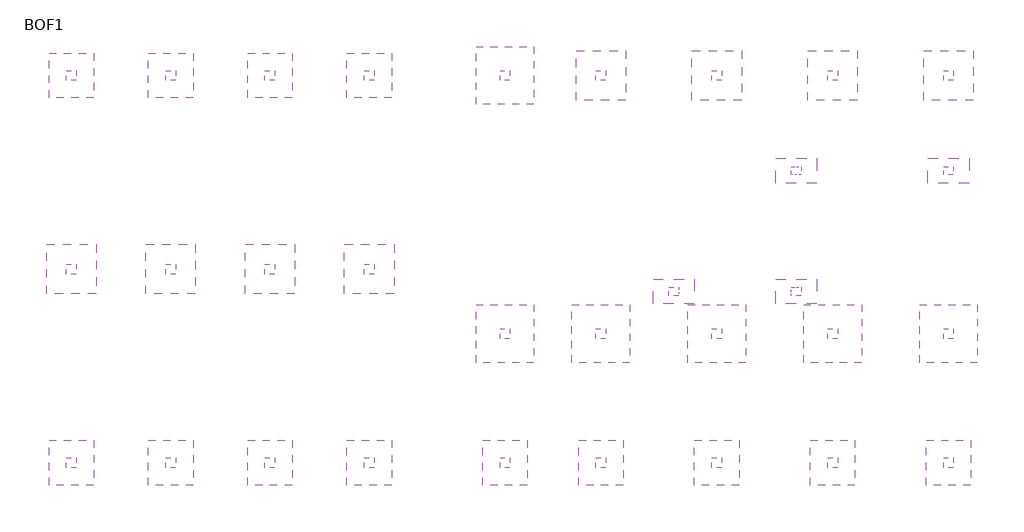
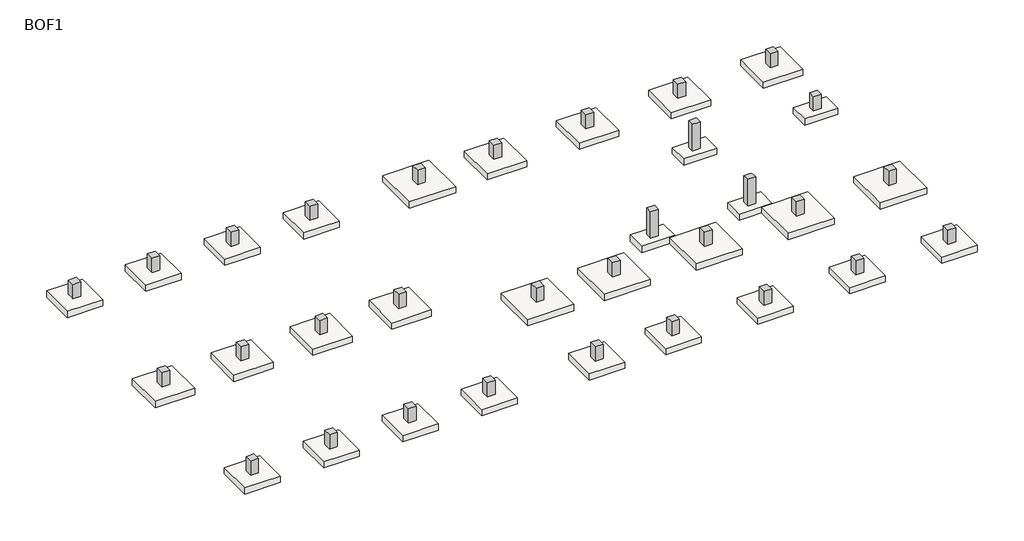
# One storey: 31 columns, 31 slabs.
"""IFC4 building model written with IfcOpenShell, lengths in millimetres."""

import ifcopenshell
import ifcopenshell.guid

model = None  # the IFC model being written
_history = None  # IfcOwnerHistory: only IFC2X3 demands one
_inside = {}  # id of a spatial element -> (the spatial element, [elements in it])
_under = {}  # id of a project, library or spatial element -> (it, [spatial elements below it])
_declared = {}  # id of a project -> (the project, [libraries it declares])
_typed = {}  # id of a type object -> (the type object, [elements of that type])
_made_of = {}  # id of a material, layer set ... -> (it, [elements and type objects made of it])


def new_model(schema):
    """Start an empty IFC model of exactly this schema.

    Asked for "IFC4X3", IfcOpenShell would pick the latest addendum, in which some entities
    have other attributes; the version numbers below select the first issue.
    IFC2X3 requires an IfcOwnerHistory on every rooted entity: one is made here for all.
    """
    global model, _history
    if schema == "IFC4X3":
        model = ifcopenshell.file(schema_version=(4, 3, 0, 0))
    else:
        model = ifcopenshell.file(schema=schema)
    _inside.clear()
    _under.clear()
    _declared.clear()
    _typed.clear()
    _made_of.clear()
    _history = None
    if model.schema == "IFC2X3":
        org = make("IfcOrganization", Name="unknown")
        user = make(
            "IfcPersonAndOrganization",
            ThePerson=make("IfcPerson", FamilyName="unknown"),
            TheOrganization=org,
        )
        app = make(
            "IfcApplication",
            ApplicationDeveloper=org,
            Version="unknown",
            ApplicationFullName="unknown",
            ApplicationIdentifier="unknown",
        )
        _history = make(
            "IfcOwnerHistory",
            OwningUser=user,
            OwningApplication=app,
            ChangeAction="ADDED",
            CreationDate=0,
        )
    return model


def make(cls, **values):
    """One entity of the class cls with the attributes given. An attribute that is None is left unset."""
    return model.create_entity(
        cls, **{name: value for name, value in values.items() if value is not None}
    )


def rooted(cls, **values):
    """An entity with a GlobalId (a new one), such as an element, a storey or a relation."""
    return make(cls, GlobalId=ifcopenshell.guid.new(), OwnerHistory=_history, **values)


def si_unit(unit_type, name, prefix=None):
    """IfcSIUnit, for example si_unit("LENGTHUNIT", "METRE", prefix="MILLI")."""
    return make("IfcSIUnit", UnitType=unit_type, Prefix=prefix, Name=name)


def assignment(units):
    """IfcUnitAssignment: the units of a project."""
    return None if units is None else make("IfcUnitAssignment", Units=units)


def point(xyz):
    """IfcCartesianPoint."""
    return None if xyz is None else make("IfcCartesianPoint", Coordinates=xyz)


def direction(xyz):
    """IfcDirection."""
    return None if xyz is None else make("IfcDirection", DirectionRatios=xyz)


def frame(location, z_axis=None, x_axis=None):
    """IfcAxis2Placement3D, a coordinate frame: its origin and axes. An axis left out is left unset."""
    return make(
        "IfcAxis2Placement3D",
        Location=point(location),
        Axis=direction(z_axis),
        RefDirection=direction(x_axis),
    )


def origin():
    """The frame at (0, 0, 0) with its axes left unset."""
    return frame((0.0, 0.0, 0.0))


def place(relative_to, where):
    """IfcLocalPlacement: puts the frame where relative to a parent placement (None: the world)."""
    return make(
        "IfcLocalPlacement", PlacementRelTo=relative_to, RelativePlacement=where
    )


def context(
    kind, dimensions, precision=None, world=None, true_north=None, identifier=None
):
    """IfcGeometricRepresentationContext, for example the 3D "Model" context."""
    return make(
        "IfcGeometricRepresentationContext",
        ContextIdentifier=identifier,
        ContextType=kind,
        CoordinateSpaceDimension=dimensions,
        Precision=precision,
        WorldCoordinateSystem=world,
        TrueNorth=true_north,
    )


def project(units=None, contexts=None):
    """IfcProject with its units and contexts."""
    return rooted(
        "IfcProject",
        Name="project",
        RepresentationContexts=contexts,
        UnitsInContext=assignment(units),
    )


def spatial(cls, under=None, at=None, **own):
    """A site, building, storey or space (cls), placed at a placement, below another one or the project."""
    s = rooted(cls, ObjectPlacement=at, **own)
    if under is not None:
        _under.setdefault(under.id(), (under, []))[1].append(s)
    return s


def polyline(points):
    """IfcPolyline through the points."""
    return make("IfcPolyline", Points=[point(p) for p in points])


def outline(outer, holes=None, kind="AREA"):
    """IfcArbitraryClosedProfileDef: a profile drawn as a closed curve; with holes, ...WithVoids."""
    if holes is None:
        return make("IfcArbitraryClosedProfileDef", ProfileType=kind, OuterCurve=outer)
    return make(
        "IfcArbitraryProfileDefWithVoids",
        ProfileType=kind,
        OuterCurve=outer,
        InnerCurves=holes,
    )


def extrude(swept, where, along, depth):
    """IfcExtrudedAreaSolid: the profile swept, set in the frame where, extruded along a direction by depth."""
    return make(
        "IfcExtrudedAreaSolid",
        SweptArea=swept,
        Position=where,
        ExtrudedDirection=direction(along),
        Depth=depth,
    )


def faces_of(points, faces, orient=None, outer=None):
    """IfcFace entities. A face is a list of loops; a loop is a list of indices into points, from 0.

    orient and outer hold one flag for each loop. By default every Orientation is true, the
    first loop of a face is its IfcFaceOuterBound and the others are IfcFaceBound.
    """
    made = []
    for i, loops in enumerate(faces):
        bounds = []
        for j, loop in enumerate(loops):
            is_outer = j == 0 if outer is None else outer[i][j]
            bounds.append(
                make(
                    "IfcFaceOuterBound" if is_outer else "IfcFaceBound",
                    Bound=make("IfcPolyLoop", Polygon=[points[k] for k in loop]),
                    Orientation=True if orient is None else orient[i][j],
                )
            )
        made.append(make("IfcFace", Bounds=bounds))
    return made


def faceted_brep(points, faces, orient=None, outer=None, voids=None):
    """IfcFacetedBrep: a solid bounded by flat faces; with voids (closed shells), ...WithVoids."""
    shared = [point(p) for p in points]
    hull = make("IfcClosedShell", CfsFaces=faces_of(shared, faces, orient, outer))
    if voids is None:
        return make("IfcFacetedBrep", Outer=hull)
    return make(
        "IfcFacetedBrepWithVoids",
        Outer=hull,
        Voids=[
            make(cls, CfsFaces=faces_of(shared, fs, o, b)) for cls, fs, o, b in voids
        ],
    )


def shape(context_of_items, identifier, shape_type, items):
    """IfcShapeRepresentation: the items that make up one representation, for example the "Body"."""
    return make(
        "IfcShapeRepresentation",
        ContextOfItems=context_of_items,
        RepresentationIdentifier=identifier,
        RepresentationType=shape_type,
        Items=items,
    )


def source(mapping_origin, context_of_items, identifier, shape_type, items):
    """IfcRepresentationMap: a shape defined once, which mapped items show again and again."""
    return make(
        "IfcRepresentationMap",
        MappingOrigin=mapping_origin,
        MappedRepresentation=shape(context_of_items, identifier, shape_type, items),
    )


def transform(
    local_origin,
    x_axis=None,
    y_axis=None,
    z_axis=None,
    scale=None,
    scale2=None,
    scale3=None,
    uniform=True,
):
    """IfcCartesianTransformationOperator3D, or its non-uniform kind. x_axis, y_axis, z_axis: its Axis1, 2, 3."""
    if uniform:
        return make(
            "IfcCartesianTransformationOperator3D",
            Axis1=direction(x_axis),
            Axis2=direction(y_axis),
            LocalOrigin=point(local_origin),
            Scale=scale,
            Axis3=direction(z_axis),
        )
    return make(
        "IfcCartesianTransformationOperator3DnonUniform",
        Axis1=direction(x_axis),
        Axis2=direction(y_axis),
        LocalOrigin=point(local_origin),
        Scale=scale,
        Axis3=direction(z_axis),
        Scale2=scale2,
        Scale3=scale3,
    )


def mapped(mapping_source, mapping_target):
    """IfcMappedItem: shows the shape of a source again, moved by a transform."""
    return make(
        "IfcMappedItem", MappingSource=mapping_source, MappingTarget=mapping_target
    )


def made_of(thing, what):
    """Note that an element or type object is made of a material, layer set ...; save() writes the relation."""
    if what is not None:
        _made_of.setdefault(what.id(), (what, []))[1].append(thing)
    return thing


def element(
    cls,
    number,
    at=None,
    inside=None,
    cuts=None,
    type_object=None,
    material=None,
    context=None,
    identifier="Body",
    shape_type=None,
    held_by="IfcProductDefinitionShape",
    body=None,
    shapes=None,
    **own,
):
    """One element of the class cls, such as IfcWall. Its Tag is "e" and its number.

    at: its placement. inside: the storey or other place that contains it. cuts: it is an
    opening in that element (IfcRelVoidsElement). A single representation is given by context,
    identifier, shape_type and body (its items); several are given by shapes. held_by: the class
    of the entity that holds the representations. save() writes the other relations.
    """
    e = rooted(cls, Tag="e%d" % number, ObjectPlacement=at, **own)
    if body is not None:
        shapes = [shape(context, identifier, shape_type, body)]
    if shapes is not None:
        e.Representation = make(held_by, Representations=shapes)
    if inside is not None:
        _inside.setdefault(inside.id(), (inside, []))[1].append(e)
    if cuts is not None:
        rooted(
            "IfcRelVoidsElement", RelatingBuildingElement=cuts, RelatedOpeningElement=e
        )
    if type_object is not None:
        _typed.setdefault(type_object.id(), (type_object, []))[1].append(e)
    return made_of(e, material)


def aggregate(whole, parts):
    """IfcRelAggregates: a whole, such as a stair, and the parts it consists of."""
    return rooted("IfcRelAggregates", RelatingObject=whole, RelatedObjects=parts)


def save(model, path):
    """Write the relations noted so far, then the file.

    IfcRelAggregates (storeys below a building ...), IfcRelContainedInSpatialStructure (elements
    in a storey), IfcRelDefinesByType, IfcRelAssociatesMaterial and IfcRelDeclares: one each for
    every whole, place, type object, material and project.
    """
    for whole, parts in _under.values():
        aggregate(whole, parts)
    for where, things in _inside.values():
        rooted(
            "IfcRelContainedInSpatialStructure",
            RelatedElements=things,
            RelatingStructure=where,
        )
    for kind, things in _typed.values():
        rooted("IfcRelDefinesByType", RelatedObjects=things, RelatingType=kind)
    for what, things in _made_of.values():
        rooted("IfcRelAssociatesMaterial", RelatedObjects=things, RelatingMaterial=what)
    for by, libraries in _declared.values():
        rooted("IfcRelDeclares", RelatingContext=by, RelatedDefinitions=libraries)
    model.write(path)


def foundation_rectangular_non_pile_db20e422(model_context):
    return source(origin(), model_context, "Body", "SweptSolid", [
        extrude(outline(polyline([(1350.0, 1350.0), (1350.0, -1350.0), (-1350.0, -1350.0), (-1350.0, 1350.0), (1350.0, 1350.0)])), frame((0.0, 0.0, -500.0), z_axis=(0.0, 0.0, 1.0), x_axis=(1.0, 0.0, 0.0)), (0.0, 0.0, 1.0), 500.0),
    ])


def foundation_rectangular_non_pile_a43cc813(model_context):
    return source(origin(), model_context, "Body", "SweptSolid", [
        extrude(outline(polyline([(1500.0, 1500.0), (1500.0, -1500.0), (-1500.0, -1500.0), (-1500.0, 1500.0), (1500.0, 1500.0)])), frame((0.0, 0.0, -500.0), z_axis=(0.0, 0.0, 1.0), x_axis=(1.0, 0.0, 0.0)), (0.0, 0.0, 1.0), 500.0),
    ])


def foundation_rectangular_non_pile_20b31725(model_context):
    return source(origin(), model_context, "Body", "SweptSolid", [
        extrude(outline(polyline([(1750.0, 1750.0), (1750.0, -1750.0), (-1750.0, -1750.0), (-1750.0, 1750.0), (1750.0, 1750.0)])), frame((0.0, 0.0, -500.0), z_axis=(0.0, 0.0, 1.0), x_axis=(1.0, 0.0, 0.0)), (0.0, 0.0, 1.0), 500.0),
    ])


def foundation_rectangular_non_pile_907a7f09(model_context):
    return source(origin(), model_context, "Body", "SweptSolid", [
        extrude(outline(polyline([(1250.0, 750.0), (1250.0, -750.0), (-1250.0, -750.0), (-1250.0, 750.0), (1250.0, 750.0)])), frame((0.0, 0.0, -500.0), z_axis=(0.0, 0.0, 1.0), x_axis=(1.0, 0.0, 0.0)), (0.0, 0.0, 1.0), 500.0),
    ])


model = new_model("IFC4")

# Units and contexts
model_context = context("Model", 3, world=origin())
ifc_project = project(units=[si_unit("LENGTHUNIT", "METRE", prefix="MILLI")], contexts=[model_context])

# Site, building, storey
site = spatial("IfcSite", under=ifc_project)
building = spatial("IfcBuilding", under=site)
storey = spatial("IfcBuildingStorey", under=building, Name="BOF1", Elevation=88650.0)

# Columns
placement = place(None, origin())
element("IfcColumn", 1, ObjectType="RC_Column_Rectangular : H_SC_AR_S15_UG PED_Bit_600x500_PD1", at=placement, inside=storey, context=model_context, shape_type="Brep", body=[
    faceted_brep([(36700.0, -9400.0, 95900.0), (36100.0, -9400.0, 95900.0), (36100.0, -8900.0, 95900.0), (36700.0, -8900.0, 95900.0), (36700.0, -9400.0, 98049.9618634), (36100.0, -9400.0, 98049.9618634), (36700.0, -9400.0, 97049.9618634), (36100.0, -8900.0, 98049.9618634), (36700.0, -8900.0, 98049.9618634), (36700.0, -9200.0, 98049.9618634)], [[[0, 1, 2, 3]], [[4, 5, 1, 0, 6]], [[5, 7, 2, 1]], [[7, 8, 3, 2]], [[8, 9, 4, 6, 0, 3]], [[4, 9, 8, 7, 5]]]),
])
element("IfcColumn", 2, ObjectType="RC_Column_Rectangular : H_SC_AR_S15_UG PED_Bit_600x500_PD1", at=placement, inside=storey, context=model_context, shape_type="Brep", body=[
    faceted_brep([(44100.0, -9400.0, 95900.0), (43500.0, -9400.0, 95900.0), (43500.0, -8900.0, 95900.0), (44100.0, -8900.0, 95900.0), (44100.0, -9400.0, 98049.9618634), (43500.0, -9400.0, 98049.9618634), (43500.0, -9400.0, 97049.9618634), (43500.0, -9200.0, 98049.9618634), (43500.0, -8900.0, 98049.9618634), (43600.0, -8900.0, 98049.9618634), (43800.0, -8900.0, 98049.9618634), (44100.0, -8900.0, 98049.9618634)], [[[0, 1, 2, 3]], [[4, 5, 6, 1, 0]], [[5, 7, 8, 2, 1, 6]], [[8, 9, 10, 11, 3, 2]], [[11, 4, 0, 3]], [[4, 11, 10, 9, 8, 7, 5]]]),
])
element("IfcColumn", 3, ObjectType="RC_Column_Rectangular : H_SC_AR_S15_UG PED_Bit_600x500_PD1", at=placement, inside=storey, context=model_context, shape_type="Brep", body=[
    faceted_brep([(44100.0, -2100.0, 95900.0), (43500.0, -2100.0, 95900.0), (43500.0, -1600.0, 95900.0), (44100.0, -1600.0, 95900.0), (44100.0, -2100.0, 98049.9618634), (43800.0, -2100.0, 98049.9618634), (43600.0, -2100.0, 98049.9618634), (43500.0, -2100.0, 98049.9618634), (43500.0, -2100.0, 97049.9618634), (43500.0, -2100.0, 96399.9618634), (44100.0, -2100.0, 96399.9618634), (44100.0, -2100.0, 97049.9618634), (43500.0, -1600.0, 98049.9618634), (43500.0, -1600.0, 97049.9618634), (43500.0, -1600.0, 96399.9618634), (43600.0, -1600.0, 98049.9618634), (43800.0, -1600.0, 98049.9618634), (44100.0, -1600.0, 98049.9618634), (44100.0, -1600.0, 97049.9618634), (44100.0, -1600.0, 96399.9618634)], [[[0, 1, 2, 3]], [[4, 5, 6, 7, 8, 9, 1, 0, 10, 11]], [[7, 12, 13, 14, 2, 1, 9, 8]], [[12, 15, 16, 17, 18, 19, 3, 2, 14, 13]], [[17, 4, 11, 10, 0, 3, 19, 18]], [[4, 17, 16, 15, 12, 7, 6, 5]]]),
])
element("IfcColumn", 4, ObjectType="RC_Column_Rectangular : H_SC_AR_S15_UG PED_Bit_600x500_PD1A", at=placement, inside=storey, context=model_context, shape_type="Brep", body=[
    faceted_brep([(53300.0, -2100.0, 95900.0), (52700.0, -2100.0, 95900.0), (52700.0, -1600.0, 95900.0), (53300.0, -1600.0, 95900.0), (53300.0, -2100.0, 97049.9618634), (52700.0, -2100.0, 97049.9618634), (52700.0, -2100.0, 96399.9618634), (53300.0, -2100.0, 96399.9618634), (52700.0, -1600.0, 97049.9618634), (52700.0, -1600.0, 96399.9618634), (53300.0, -1600.0, 97049.9618634), (53300.0, -1600.0, 96399.9618634)], [[[0, 1, 2, 3]], [[4, 5, 6, 1, 0, 7]], [[5, 8, 9, 2, 1, 6]], [[8, 10, 11, 3, 2, 9]], [[10, 4, 7, 0, 3, 11]], [[4, 10, 8, 5]]]),
])
element("IfcColumn", 5, ObjectType="RC_Column_Rectangular : H_SC_AR S15_UG Ped_C1 600x600", at=placement, inside=storey, context=model_context, shape_type="SweptSolid", body=[
    extrude(outline(polyline([(300.0, -19200.0), (300.0, -19800.0), (-300.0, -19800.0), (-300.0, -19200.0), (300.0, -19200.0)])), frame((0.0, 0.0, 95900.0), z_axis=(0.0, 0.0, 1.0), x_axis=(1.0, 0.0, 0.0)), (0.0, 0.0, 1.0), 1149.9618634),
])
element("IfcColumn", 6, ObjectType="RC_Column_Rectangular : H_SC_AR S15_UG Ped_C1 600x600", at=placement, inside=storey, context=model_context, shape_type="Brep", body=[
    faceted_brep([(26500.0, -11400.0, 95900.0), (26500.0, -12000.0, 95900.0), (25900.0, -12000.0, 95900.0), (25900.0, -11400.0, 95900.0), (26500.0, -11400.0, 97049.9618634), (26500.0, -12000.0, 97049.9618634), (25900.0, -12000.0, 97049.9618634), (25900.0, -11400.0, 97049.9618634), (25900.0, -11400.0, 96849.9618634)], [[[0, 1, 2, 3]], [[4, 5, 1, 0]], [[5, 6, 2, 1]], [[6, 7, 8, 3, 2]], [[7, 4, 0, 3, 8]], [[4, 7, 6, 5]]]),
])
element("IfcColumn", 7, ObjectType="RC_Column_Rectangular : H_SC_AR S15_UG Ped_C1 600x600", at=placement, inside=storey, context=model_context, shape_type="Brep", body=[
    faceted_brep([(300.0, -7500.0, 95900.0), (300.0, -8100.0, 95900.0), (-300.0, -8100.0, 95900.0), (-300.0, -7500.0, 95900.0), (300.0, -7500.0, 97049.9618634), (300.0, -8100.0, 97049.9618634), (300.0, -8100.0, 96399.9618634), (300.0, -7500.0, 96399.9618634), (-300.0, -8100.0, 97049.9618634), (-300.0, -8100.0, 96399.9618634), (-300.0, -7500.0, 97049.9618634), (-300.0, -7500.0, 96399.9618634)], [[[0, 1, 2, 3]], [[4, 5, 6, 1, 0, 7]], [[5, 8, 9, 2, 1, 6]], [[8, 10, 11, 3, 2, 9]], [[10, 4, 7, 0, 3, 11]], [[4, 10, 8, 5]]]),
])
element("IfcColumn", 8, ObjectType="RC_Column_Rectangular : H_SC_AR S15_UG Ped_C1 600x600", at=placement, inside=storey, context=model_context, shape_type="Brep", body=[
    faceted_brep([(300.0, 4200.0, 95900.0), (300.0, 3600.0, 95900.0), (-300.0, 3600.0, 95900.0), (-300.0, 4200.0, 95900.0), (300.0, 4200.0, 97049.9618634), (300.0, 3600.0, 97049.9618634), (300.0, 3600.0, 96399.9618634), (300.0, 4200.0, 96399.9618634), (-300.0, 3600.0, 97049.9618634), (-300.0, 3600.0, 96399.9618634), (-300.0, 4200.0, 97049.9618634)], [[[0, 1, 2, 3]], [[4, 5, 6, 1, 0, 7]], [[5, 8, 9, 2, 1, 6]], [[8, 10, 3, 2, 9]], [[10, 4, 7, 0, 3]], [[4, 10, 8, 5]]]),
])
element("IfcColumn", 9, ObjectType="RC_Column_Rectangular : H_SC_AR S15_UG Ped_C1 600x600", at=placement, inside=storey, context=model_context, shape_type="Brep", body=[
    faceted_brep([(26500.0, -19200.0, 95900.0), (26500.0, -19800.0, 95900.0), (25900.0, -19800.0, 95900.0), (25900.0, -19200.0, 95900.0), (26500.0, -19200.0, 97049.9618634), (26500.0, -19800.0, 97049.9618634), (26500.0, -19800.0, 96399.9618634), (26500.0, -19200.0, 96399.9618634), (25900.0, -19800.0, 97049.9618634), (25900.0, -19800.0, 96399.9618634), (25900.0, -19200.0, 97049.9618634), (25900.0, -19200.0, 96399.9618634)], [[[0, 1, 2, 3]], [[4, 5, 6, 1, 0, 7]], [[5, 8, 9, 2, 1, 6]], [[8, 10, 11, 3, 2, 9]], [[10, 4, 7, 0, 3, 11]], [[4, 10, 8, 5]]]),
])
element("IfcColumn", 10, ObjectType="RC_Column_Rectangular : H_SC_AR S15_UG Ped_C1 600x600", at=placement, inside=storey, context=model_context, shape_type="Brep", body=[
    faceted_brep([(32300.0, -19200.0, 95900.0), (32300.0, -19800.0, 95900.0), (31700.0, -19800.0, 95900.0), (31700.0, -19200.0, 95900.0), (32300.0, -19200.0, 97049.9618634), (32300.0, -19800.0, 97049.9618634), (32300.0, -19800.0, 96399.9618634), (32300.0, -19200.0, 96399.9618634), (31700.0, -19800.0, 97049.9618634), (31700.0, -19800.0, 96399.9618634), (31700.0, -19200.0, 97049.9618634), (31700.0, -19200.0, 96399.9618634)], [[[0, 1, 2, 3]], [[4, 5, 6, 1, 0, 7]], [[5, 8, 9, 2, 1, 6]], [[8, 10, 11, 3, 2, 9]], [[10, 4, 7, 0, 3, 11]], [[4, 10, 8, 5]]]),
])
element("IfcColumn", 11, ObjectType="RC_Column_Rectangular : H_SC_AR S15_UG Ped_C1 600x600", at=placement, inside=storey, context=model_context, shape_type="Brep", body=[
    faceted_brep([(39300.0, -19200.0, 95900.0), (39300.0, -19800.0, 95900.0), (38700.0, -19800.0, 95900.0), (38700.0, -19200.0, 95900.0), (39300.0, -19200.0, 97049.9618634), (39300.0, -19800.0, 97049.9618634), (39300.0, -19800.0, 96399.9618634), (39300.0, -19200.0, 96399.9618634), (38700.0, -19800.0, 97049.9618634), (38700.0, -19800.0, 96399.9618634), (38700.0, -19200.0, 97049.9618634), (38700.0, -19200.0, 96399.9618634)], [[[0, 1, 2, 3]], [[4, 5, 6, 1, 0, 7]], [[5, 8, 9, 2, 1, 6]], [[8, 10, 11, 3, 2, 9]], [[10, 4, 7, 0, 3, 11]], [[4, 10, 8, 5]]]),
])
element("IfcColumn", 12, ObjectType="RC_Column_Rectangular : H_SC_AR S15_UG Ped_C1 600x600", at=placement, inside=storey, context=model_context, shape_type="Brep", body=[
    faceted_brep([(46300.0, -19200.0, 95900.0), (46300.0, -19800.0, 95900.0), (45700.0, -19800.0, 95900.0), (45700.0, -19200.0, 95900.0), (46300.0, -19200.0, 97049.9618634), (46300.0, -19800.0, 97049.9618634), (46300.0, -19800.0, 96399.9618634), (46300.0, -19200.0, 96399.9618634), (45700.0, -19800.0, 97049.9618634), (45700.0, -19800.0, 96399.9618634), (45700.0, -19200.0, 97049.9618634), (45700.0, -19200.0, 96399.9618634)], [[[0, 1, 2, 3]], [[4, 5, 6, 1, 0, 7]], [[5, 8, 9, 2, 1, 6]], [[8, 10, 11, 3, 2, 9]], [[10, 4, 7, 0, 3, 11]], [[4, 10, 8, 5]]]),
])
element("IfcColumn", 13, ObjectType="RC_Column_Rectangular : H_SC_AR S15_UG Ped_C1 600x600", at=placement, inside=storey, context=model_context, shape_type="Brep", body=[
    faceted_brep([(53300.0, -19200.0, 95900.0), (53300.0, -19800.0, 95900.0), (52700.0, -19800.0, 95900.0), (52700.0, -19200.0, 95900.0), (53300.0, -19200.0, 97049.9618634), (53300.0, -19800.0, 97049.9618634), (53300.0, -19200.0, 96399.9618634), (52700.0, -19800.0, 97049.9618634), (52700.0, -19800.0, 96399.9618634), (52700.0, -19200.0, 97049.9618634), (52700.0, -19200.0, 96399.9618634)], [[[0, 1, 2, 3]], [[4, 5, 1, 0, 6]], [[5, 7, 8, 2, 1]], [[7, 9, 10, 3, 2, 8]], [[9, 4, 6, 0, 3, 10]], [[4, 9, 7, 5]]]),
])
element("IfcColumn", 14, ObjectType="RC_Column_Rectangular : H_SC_AR S15_UG Ped_C1 600x600", at=placement, inside=storey, context=model_context, shape_type="Brep", body=[
    faceted_brep([(6300.0, -19200.0, 95900.0), (6300.0, -19800.0, 95900.0), (5700.0, -19800.0, 95900.0), (5700.0, -19200.0, 95900.0), (6300.0, -19200.0, 97049.9618634), (6300.0, -19800.0, 97049.9618634), (6300.0, -19800.0, 96399.9618634), (6300.0, -19200.0, 96399.9618634), (5700.0, -19800.0, 97049.9618634), (5700.0, -19800.0, 96399.9618634), (5700.0, -19200.0, 97049.9618634), (5700.0, -19200.0, 96399.9618634)], [[[0, 1, 2, 3]], [[4, 5, 6, 1, 0, 7]], [[5, 8, 9, 2, 1, 6]], [[8, 10, 11, 3, 2, 9]], [[10, 4, 7, 0, 3, 11]], [[4, 10, 8, 5]]]),
])
element("IfcColumn", 15, ObjectType="RC_Column_Rectangular : H_SC_AR S15_UG Ped_C1 600x600", at=placement, inside=storey, context=model_context, shape_type="Brep", body=[
    faceted_brep([(6300.0, -7500.0, 95900.0), (6300.0, -8100.0, 95900.0), (5700.0, -8100.0, 95900.0), (5700.0, -7500.0, 95900.0), (6300.0, -7500.0, 97049.9618634), (6300.0, -8100.0, 97049.9618634), (6300.0, -8100.0, 96849.9618634), (6300.0, -7500.0, 96849.9618634), (5700.0, -8100.0, 97049.9618634), (5700.0, -8100.0, 96849.9618634), (5700.0, -7500.0, 97049.9618634), (5700.0, -7500.0, 96849.9618634)], [[[0, 1, 2, 3]], [[4, 5, 6, 1, 0, 7]], [[5, 8, 9, 2, 1, 6]], [[8, 10, 11, 3, 2, 9]], [[10, 4, 7, 0, 3, 11]], [[4, 10, 8, 5]]]),
])
element("IfcColumn", 16, ObjectType="RC_Column_Rectangular : H_SC_AR S15_UG Ped_C1 600x600", at=placement, inside=storey, context=model_context, shape_type="Brep", body=[
    faceted_brep([(6300.0, 4200.0, 95900.0), (6300.0, 3600.0, 95900.0), (5700.0, 3600.0, 95900.0), (5700.0, 4200.0, 95900.0), (6300.0, 4200.0, 97049.9618634), (6300.0, 3600.0, 97049.9618634), (6300.0, 3600.0, 96399.9618634), (6300.0, 4200.0, 96399.9618634), (5700.0, 3600.0, 97049.9618634), (5700.0, 3600.0, 96399.9618634), (5700.0, 4200.0, 97049.9618634), (5700.0, 4200.0, 96399.9618634)], [[[0, 1, 2, 3]], [[4, 5, 6, 1, 0, 7]], [[5, 8, 9, 2, 1, 6]], [[8, 10, 11, 3, 2, 9]], [[10, 4, 7, 0, 3, 11]], [[4, 10, 8, 5]]]),
])
element("IfcColumn", 17, ObjectType="RC_Column_Rectangular : H_SC_AR S15_UG Ped_C1 600x600", at=placement, inside=storey, context=model_context, shape_type="Brep", body=[
    faceted_brep([(12300.0, -19200.0, 95900.0), (12300.0, -19800.0, 95900.0), (11700.0, -19800.0, 95900.0), (11700.0, -19200.0, 95900.0), (12300.0, -19200.0, 97049.9618634), (12300.0, -19800.0, 97049.9618634), (12300.0, -19800.0, 96399.9618634), (12300.0, -19200.0, 96399.9618634), (11700.0, -19800.0, 97049.9618634), (11700.0, -19800.0, 96399.9618634), (11700.0, -19200.0, 97049.9618634), (11700.0, -19200.0, 96399.9618634)], [[[0, 1, 2, 3]], [[4, 5, 6, 1, 0, 7]], [[5, 8, 9, 2, 1, 6]], [[8, 10, 11, 3, 2, 9]], [[10, 4, 7, 0, 3, 11]], [[4, 10, 8, 5]]]),
])
element("IfcColumn", 18, ObjectType="RC_Column_Rectangular : H_SC_AR S15_UG Ped_C1 600x600", at=placement, inside=storey, context=model_context, shape_type="Brep", body=[
    faceted_brep([(12300.0, -7500.0, 95900.0), (12300.0, -8100.0, 95900.0), (11700.0, -8100.0, 95900.0), (11700.0, -7500.0, 95900.0), (12300.0, -7500.0, 97049.9618634), (12300.0, -8100.0, 97049.9618634), (12300.0, -8100.0, 96849.9618634), (12300.0, -7500.0, 96849.9618634), (11700.0, -8100.0, 97049.9618634), (11700.0, -8100.0, 96849.9618634), (11700.0, -7500.0, 97049.9618634), (11700.0, -7500.0, 96849.9618634)], [[[0, 1, 2, 3]], [[4, 5, 6, 1, 0, 7]], [[5, 8, 9, 2, 1, 6]], [[8, 10, 11, 3, 2, 9]], [[10, 4, 7, 0, 3, 11]], [[4, 10, 8, 5]]]),
])
element("IfcColumn", 19, ObjectType="RC_Column_Rectangular : H_SC_AR S15_UG Ped_C1 600x600", at=placement, inside=storey, context=model_context, shape_type="Brep", body=[
    faceted_brep([(12300.0, 4200.0, 95900.0), (12300.0, 3600.0, 95900.0), (11700.0, 3600.0, 95900.0), (11700.0, 4200.0, 95900.0), (12300.0, 4200.0, 97049.9618634), (12300.0, 3600.0, 97049.9618634), (12300.0, 3600.0, 96399.9618634), (12300.0, 4200.0, 96399.9618634), (11700.0, 3600.0, 97049.9618634), (11700.0, 3600.0, 96399.9618634), (11700.0, 4200.0, 97049.9618634), (11700.0, 4200.0, 96399.9618634)], [[[0, 1, 2, 3]], [[4, 5, 6, 1, 0, 7]], [[5, 8, 9, 2, 1, 6]], [[8, 10, 11, 3, 2, 9]], [[10, 4, 7, 0, 3, 11]], [[4, 10, 8, 5]]]),
])
element("IfcColumn", 20, ObjectType="RC_Column_Rectangular : H_SC_AR S15_UG Ped_C1 600x600", at=placement, inside=storey, context=model_context, shape_type="Brep", body=[
    faceted_brep([(18300.0, -19200.0, 95900.0), (18300.0, -19800.0, 95900.0), (17700.0, -19800.0, 95900.0), (17700.0, -19200.0, 95900.0), (18300.0, -19200.0, 97049.9618634), (18300.0, -19800.0, 97049.9618634), (18300.0, -19800.0, 96399.9618634), (18300.0, -19200.0, 96399.9618634), (17700.0, -19800.0, 97049.9618634), (17700.0, -19800.0, 96399.9618634), (17700.0, -19200.0, 97049.9618634), (17700.0, -19200.0, 96399.9618634)], [[[0, 1, 2, 3]], [[4, 5, 6, 1, 0, 7]], [[5, 8, 9, 2, 1, 6]], [[8, 10, 11, 3, 2, 9]], [[10, 4, 7, 0, 3, 11]], [[4, 10, 8, 5]]]),
])
element("IfcColumn", 21, ObjectType="RC_Column_Rectangular : H_SC_AR S15_UG Ped_C1 600x600", at=placement, inside=storey, context=model_context, shape_type="Brep", body=[
    faceted_brep([(18300.0, -7500.0, 95900.0), (18300.0, -8100.0, 95900.0), (17700.0, -8100.0, 95900.0), (17700.0, -7500.0, 95900.0), (18300.0, -7500.0, 97049.9618634), (18300.0, -8100.0, 97049.9618634), (18300.0, -8100.0, 96849.9618634), (18300.0, -7500.0, 96849.9618634), (17700.0, -8100.0, 97049.9618634), (17700.0, -8100.0, 96849.9618634), (17700.0, -7500.0, 97049.9618634), (17700.0, -7500.0, 96849.9618634)], [[[0, 1, 2, 3]], [[4, 5, 6, 1, 0, 7]], [[5, 8, 9, 2, 1, 6]], [[8, 10, 11, 3, 2, 9]], [[10, 4, 7, 0, 3, 11]], [[4, 10, 8, 5]]]),
])
element("IfcColumn", 22, ObjectType="RC_Column_Rectangular : H_SC_AR S15_UG Ped_C1 600x600", at=placement, inside=storey, context=model_context, shape_type="Brep", body=[
    faceted_brep([(18300.0, 4200.0, 95900.0), (18300.0, 3600.0, 95900.0), (17700.0, 3600.0, 95900.0), (17700.0, 4200.0, 95900.0), (18300.0, 4200.0, 97049.9618634), (18300.0, 3600.0, 97049.9618634), (18300.0, 3600.0, 96399.9618634), (18300.0, 4200.0, 96399.9618634), (17700.0, 3600.0, 97049.9618634), (17700.0, 3600.0, 96399.9618634), (17700.0, 4200.0, 97049.9618634), (17700.0, 4200.0, 96399.9618634)], [[[0, 1, 2, 3]], [[4, 5, 6, 1, 0, 7]], [[5, 8, 9, 2, 1, 6]], [[8, 10, 11, 3, 2, 9]], [[10, 4, 7, 0, 3, 11]], [[4, 10, 8, 5]]]),
])
element("IfcColumn", 23, ObjectType="RC_Column_Rectangular : H_SC_AR S15_UG Ped_C1 600x600", at=placement, inside=storey, context=model_context, shape_type="Brep", body=[
    faceted_brep([(32300.0, -11400.0, 95900.0), (32300.0, -12000.0, 95900.0), (31700.0, -12000.0, 95900.0), (31700.0, -11400.0, 95900.0), (32300.0, -11400.0, 97049.9618634), (32300.0, -12000.0, 97049.9618634), (32300.0, -12000.0, 96399.9618634), (32300.0, -11400.0, 96399.9618634), (31700.0, -12000.0, 97049.9618634), (31700.0, -12000.0, 96399.9618634), (31700.0, -11400.0, 97049.9618634), (31700.0, -11400.0, 96399.9618634)], [[[0, 1, 2, 3]], [[4, 5, 6, 1, 0, 7]], [[5, 8, 9, 2, 1, 6]], [[8, 10, 11, 3, 2, 9]], [[10, 4, 7, 0, 3, 11]], [[4, 10, 8, 5]]]),
])
element("IfcColumn", 24, ObjectType="RC_Column_Rectangular : H_SC_AR S15_UG Ped_C1 600x600", at=placement, inside=storey, context=model_context, shape_type="Brep", body=[
    faceted_brep([(39300.0, -11400.0, 95900.0), (39300.0, -12000.0, 95900.0), (38700.0, -12000.0, 95900.0), (38700.0, -11400.0, 95900.0), (39300.0, -11400.0, 97049.9618634), (39300.0, -12000.0, 97049.9618634), (39300.0, -12000.0, 96399.9618634), (39300.0, -11400.0, 96399.9618634), (38700.0, -12000.0, 97049.9618634), (38700.0, -12000.0, 96399.9618634), (38700.0, -11400.0, 97049.9618634), (38700.0, -11400.0, 96399.9618634)], [[[0, 1, 2, 3]], [[4, 5, 6, 1, 0, 7]], [[5, 8, 9, 2, 1, 6]], [[8, 10, 11, 3, 2, 9]], [[10, 4, 7, 0, 3, 11]], [[4, 10, 8, 5]]]),
])
element("IfcColumn", 25, ObjectType="RC_Column_Rectangular : H_SC_AR S15_UG Ped_C1 600x600", at=placement, inside=storey, context=model_context, shape_type="Brep", body=[
    faceted_brep([(46300.0, -11400.0, 95900.0), (46300.0, -12000.0, 95900.0), (45700.0, -12000.0, 95900.0), (45700.0, -11400.0, 95900.0), (46300.0, -11400.0, 97049.9618634), (46300.0, -12000.0, 97049.9618634), (46300.0, -12000.0, 96399.9618634), (46300.0, -11400.0, 96399.9618634), (45700.0, -12000.0, 97049.9618634), (45700.0, -12000.0, 96399.9618634), (45700.0, -11400.0, 97049.9618634), (45700.0, -11400.0, 96399.9618634)], [[[0, 1, 2, 3]], [[4, 5, 6, 1, 0, 7]], [[5, 8, 9, 2, 1, 6]], [[8, 10, 11, 3, 2, 9]], [[10, 4, 7, 0, 3, 11]], [[4, 10, 8, 5]]]),
])
element("IfcColumn", 26, ObjectType="RC_Column_Rectangular : H_SC_AR S15_UG Ped_C1 600x600", at=placement, inside=storey, context=model_context, shape_type="Brep", body=[
    faceted_brep([(53300.0, -11400.0, 95900.0), (53300.0, -12000.0, 95900.0), (52700.0, -12000.0, 95900.0), (52700.0, -11400.0, 95900.0), (53300.0, -11400.0, 97049.9618634), (53300.0, -12000.0, 97049.9618634), (53300.0, -12000.0, 96399.9618634), (53300.0, -11400.0, 96399.9618634), (52700.0, -12000.0, 97049.9618634), (52700.0, -12000.0, 96399.9618634), (52700.0, -11400.0, 97049.9618634), (52700.0, -11400.0, 96399.9618634)], [[[0, 1, 2, 3]], [[4, 5, 6, 1, 0, 7]], [[5, 8, 9, 2, 1, 6]], [[8, 10, 11, 3, 2, 9]], [[10, 4, 7, 0, 3, 11]], [[4, 10, 8, 5]]]),
])
element("IfcColumn", 27, ObjectType="RC_Column_Rectangular : H_SC_AR S15_UG Ped_C1 600x600", at=placement, inside=storey, context=model_context, shape_type="Brep", body=[
    faceted_brep([(53300.0, 4200.0, 95900.0), (53300.0, 3600.0, 95900.0), (52700.0, 3600.0, 95900.0), (52700.0, 4200.0, 95900.0), (53300.0, 4200.0, 97049.9618634), (53300.0, 3600.0, 97049.9618634), (53300.0, 3600.0, 96399.9618634), (52700.0, 3600.0, 97049.9618634), (52700.0, 3600.0, 96399.9618634), (52700.0, 4200.0, 97049.9618634), (52700.0, 4200.0, 96399.9618634)], [[[0, 1, 2, 3]], [[4, 5, 6, 1, 0]], [[5, 7, 8, 2, 1, 6]], [[7, 9, 10, 3, 2, 8]], [[9, 4, 0, 3, 10]], [[4, 9, 7, 5]]]),
])
element("IfcColumn", 28, ObjectType="RC_Column_Rectangular : H_SC_AR S15_UG Ped_C1 600x600", at=placement, inside=storey, context=model_context, shape_type="Brep", body=[
    faceted_brep([(46300.0, 4200.0, 95900.0), (46300.0, 3600.0, 95900.0), (45700.0, 3600.0, 95900.0), (45700.0, 4200.0, 95900.0), (46300.0, 4200.0, 97049.9618634), (46300.0, 3600.0, 97049.9618634), (46300.0, 3600.0, 96399.9618634), (46300.0, 4200.0, 96399.9618634), (45700.0, 3600.0, 97049.9618634), (45700.0, 3600.0, 96399.9618634), (45700.0, 4200.0, 97049.9618634), (45700.0, 4200.0, 96399.9618634)], [[[0, 1, 2, 3]], [[4, 5, 6, 1, 0, 7]], [[5, 8, 9, 2, 1, 6]], [[8, 10, 11, 3, 2, 9]], [[10, 4, 7, 0, 3, 11]], [[4, 10, 8, 5]]]),
])
element("IfcColumn", 29, ObjectType="RC_Column_Rectangular : H_SC_AR S15_UG Ped_C1 600x600", at=placement, inside=storey, context=model_context, shape_type="Brep", body=[
    faceted_brep([(39300.0, 4200.0, 95900.0), (39300.0, 3600.0, 95900.0), (38700.0, 3600.0, 95900.0), (38700.0, 4200.0, 95900.0), (39300.0, 4200.0, 97049.9618634), (39300.0, 3600.0, 97049.9618634), (39300.0, 3600.0, 96399.9618634), (39300.0, 4200.0, 96399.9618634), (38700.0, 3600.0, 97049.9618634), (38700.0, 3600.0, 96399.9618634), (38700.0, 4200.0, 97049.9618634), (38700.0, 4200.0, 96399.9618634)], [[[0, 1, 2, 3]], [[4, 5, 6, 1, 0, 7]], [[5, 8, 9, 2, 1, 6]], [[8, 10, 11, 3, 2, 9]], [[10, 4, 7, 0, 3, 11]], [[4, 10, 8, 5]]]),
])
element("IfcColumn", 30, ObjectType="RC_Column_Rectangular : H_SC_AR S15_UG Ped_C1 600x600", at=placement, inside=storey, context=model_context, shape_type="Brep", body=[
    faceted_brep([(32300.0, 4200.0, 95900.0), (32300.0, 3600.0, 95900.0), (31700.0, 3600.0, 95900.0), (31700.0, 4200.0, 95900.0), (32300.0, 4200.0, 97049.9618634), (32300.0, 3600.0, 97049.9618634), (32300.0, 3600.0, 96399.9618634), (32300.0, 4200.0, 96399.9618634), (31700.0, 3600.0, 97049.9618634), (31700.0, 3600.0, 96399.9618634), (31700.0, 4200.0, 97049.9618634), (31700.0, 4200.0, 96399.9618634)], [[[0, 1, 2, 3]], [[4, 5, 6, 1, 0, 7]], [[5, 8, 9, 2, 1, 6]], [[8, 10, 11, 3, 2, 9]], [[10, 4, 7, 0, 3, 11]], [[4, 10, 8, 5]]]),
])
element("IfcColumn", 31, ObjectType="RC_Column_Rectangular : H_SC_AR S15_UG Ped_C1 600x600", at=placement, inside=storey, context=model_context, shape_type="Brep", body=[
    faceted_brep([(26500.0, 4200.0, 95900.0), (26500.0, 3600.0, 95900.0), (25900.0, 3600.0, 95900.0), (25900.0, 4200.0, 95900.0), (26500.0, 4200.0, 97049.9618634), (26500.0, 3600.0, 97049.9618634), (26500.0, 3600.0, 96399.9618634), (26500.0, 4200.0, 96399.9618634), (25900.0, 3600.0, 97049.9618634), (25900.0, 3600.0, 96399.9618634), (25900.0, 4200.0, 97049.9618634), (25900.0, 4200.0, 96399.9618634)], [[[0, 1, 2, 3]], [[4, 5, 6, 1, 0, 7]], [[5, 8, 9, 2, 1, 6]], [[8, 10, 11, 3, 2, 9]], [[10, 4, 7, 0, 3, 11]], [[4, 10, 8, 5]]]),
])

# Slabs
element("IfcSlab", 32, ObjectType="Foundation Rectangular (Non-Pile) : H_SF_AR S18_Ret Fdn_F4 2500x1500x500", at=placement, inside=storey, context=model_context, shape_type="SweptSolid", body=[
    extrude(outline(polyline([(45050.0, -1100.0), (45050.0, -2600.0), (42550.0, -2600.0), (42550.0, -1100.0), (45050.0, -1100.0)])), frame((0.0, 0.0, 95400.0), z_axis=(0.0, 0.0, 1.0), x_axis=(1.0, 0.0, 0.0)), (0.0, 0.0, 1.0), 500.0),
])
foundation_rectangular_non_pile_shape = foundation_rectangular_non_pile_db20e422(model_context)
element("IfcSlab", 33, ObjectType="Foundation Rectangular (Non-Pile) : H_SF_AR S18_Ret Fdn_F1 2700x2700x500", at=placement, inside=storey, context=model_context, shape_type="MappedRepresentation", body=[
    mapped(foundation_rectangular_non_pile_shape, transform((0.0, 3900.0, 95900.0), x_axis=(1.0, 0.0, 0.0), y_axis=(0.0, 1.0, 0.0), z_axis=(0.0, 0.0, 1.0))),
])
element("IfcSlab", 34, ObjectType="Foundation Rectangular (Non-Pile) : H_SF_AR S18_Ret Fdn_F1 2700x2700x500", at=placement, inside=storey, context=model_context, shape_type="MappedRepresentation", body=[
    mapped(foundation_rectangular_non_pile_shape, transform((6000.0, 3900.0, 95900.0), x_axis=(1.0, 0.0, 0.0), y_axis=(0.0, 1.0, 0.0), z_axis=(0.0, 0.0, 1.0))),
])
element("IfcSlab", 35, ObjectType="Foundation Rectangular (Non-Pile) : H_SF_AR S18_Ret Fdn_F1 2700x2700x500", at=placement, inside=storey, context=model_context, shape_type="MappedRepresentation", body=[
    mapped(foundation_rectangular_non_pile_shape, transform((12000.0, 3900.0, 95900.0), x_axis=(1.0, 0.0, 0.0), y_axis=(0.0, 1.0, 0.0), z_axis=(0.0, 0.0, 1.0))),
])
element("IfcSlab", 36, ObjectType="Foundation Rectangular (Non-Pile) : H_SF_AR S18_Ret Fdn_F1 2700x2700x500", at=placement, inside=storey, context=model_context, shape_type="MappedRepresentation", body=[
    mapped(foundation_rectangular_non_pile_shape, transform((18000.0, 3900.0, 95900.0), x_axis=(1.0, 0.0, 0.0), y_axis=(0.0, 1.0, 0.0), z_axis=(0.0, 0.0, 1.0))),
])
element("IfcSlab", 37, ObjectType="Foundation Rectangular (Non-Pile) : H_SF_AR S18_Ret Fdn_F1 2700x2700x500", at=placement, inside=storey, context=model_context, shape_type="MappedRepresentation", body=[
    mapped(foundation_rectangular_non_pile_shape, transform((0.0, -19500.0, 95900.0), x_axis=(1.0, 0.0, 0.0), y_axis=(0.0, 1.0, 0.0), z_axis=(0.0, 0.0, 1.0))),
])
element("IfcSlab", 38, ObjectType="Foundation Rectangular (Non-Pile) : H_SF_AR S18_Ret Fdn_F1 2700x2700x500", at=placement, inside=storey, context=model_context, shape_type="MappedRepresentation", body=[
    mapped(foundation_rectangular_non_pile_shape, transform((6000.0, -19500.0, 95900.0), x_axis=(1.0, 0.0, 0.0), y_axis=(0.0, 1.0, 0.0), z_axis=(0.0, 0.0, 1.0))),
])
element("IfcSlab", 39, ObjectType="Foundation Rectangular (Non-Pile) : H_SF_AR S18_Ret Fdn_F1 2700x2700x500", at=placement, inside=storey, context=model_context, shape_type="MappedRepresentation", body=[
    mapped(foundation_rectangular_non_pile_shape, transform((12000.0, -19500.0, 95900.0), x_axis=(1.0, 0.0, 0.0), y_axis=(0.0, 1.0, 0.0), z_axis=(0.0, 0.0, 1.0))),
])
element("IfcSlab", 40, ObjectType="Foundation Rectangular (Non-Pile) : H_SF_AR S18_Ret Fdn_F1 2700x2700x500", at=placement, inside=storey, context=model_context, shape_type="MappedRepresentation", body=[
    mapped(foundation_rectangular_non_pile_shape, transform((18000.0, -19500.0, 95900.0), x_axis=(1.0, 0.0, 0.0), y_axis=(0.0, 1.0, 0.0), z_axis=(0.0, 0.0, 1.0))),
])
element("IfcSlab", 41, ObjectType="Foundation Rectangular (Non-Pile) : H_SF_AR S18_Ret Fdn_F1 2700x2700x500", at=placement, inside=storey, context=model_context, shape_type="MappedRepresentation", body=[
    mapped(foundation_rectangular_non_pile_shape, transform((26200.0, -19500.0, 95900.0), x_axis=(1.0, 0.0, 0.0), y_axis=(0.0, 1.0, 0.0), z_axis=(0.0, 0.0, 1.0))),
])
element("IfcSlab", 42, ObjectType="Foundation Rectangular (Non-Pile) : H_SF_AR S18_Ret Fdn_F1 2700x2700x500", at=placement, inside=storey, context=model_context, shape_type="MappedRepresentation", body=[
    mapped(foundation_rectangular_non_pile_shape, transform((32000.0, -19500.0, 95900.0), x_axis=(1.0, 0.0, 0.0), y_axis=(0.0, 1.0, 0.0), z_axis=(0.0, 0.0, 1.0))),
])
element("IfcSlab", 43, ObjectType="Foundation Rectangular (Non-Pile) : H_SF_AR S18_Ret Fdn_F1 2700x2700x500", at=placement, inside=storey, context=model_context, shape_type="MappedRepresentation", body=[
    mapped(foundation_rectangular_non_pile_shape, transform((39000.0, -19500.0, 95900.0), x_axis=(1.0, 0.0, 0.0), y_axis=(0.0, 1.0, 0.0), z_axis=(0.0, 0.0, 1.0))),
])
element("IfcSlab", 44, ObjectType="Foundation Rectangular (Non-Pile) : H_SF_AR S18_Ret Fdn_F1 2700x2700x500", at=placement, inside=storey, context=model_context, shape_type="MappedRepresentation", body=[
    mapped(foundation_rectangular_non_pile_shape, transform((46000.0, -19500.0, 95900.0), x_axis=(1.0, 0.0, 0.0), y_axis=(0.0, 1.0, 0.0), z_axis=(0.0, 0.0, 1.0))),
])
element("IfcSlab", 45, ObjectType="Foundation Rectangular (Non-Pile) : H_SF_AR S18_Ret Fdn_F1 2700x2700x500", at=placement, inside=storey, context=model_context, shape_type="MappedRepresentation", body=[
    mapped(foundation_rectangular_non_pile_shape, transform((53000.0, -19500.0, 95900.0), x_axis=(1.0, 0.0, 0.0), y_axis=(0.0, 1.0, 0.0), z_axis=(0.0, 0.0, 1.0))),
])
foundation_rectangular_non_pile_2_shape = foundation_rectangular_non_pile_a43cc813(model_context)
element("IfcSlab", 46, ObjectType="Foundation Rectangular (Non-Pile) : H_SF_AR S18_Ret Fdn_F2 3000x3000x500", at=placement, inside=storey, context=model_context, shape_type="MappedRepresentation", body=[
    mapped(foundation_rectangular_non_pile_2_shape, transform((32000.0, 3900.0, 95900.0), x_axis=(1.0, 0.0, 0.0), y_axis=(0.0, 1.0, 0.0), z_axis=(0.0, 0.0, 1.0))),
])
element("IfcSlab", 47, ObjectType="Foundation Rectangular (Non-Pile) : H_SF_AR S18_Ret Fdn_F2 3000x3000x500", at=placement, inside=storey, context=model_context, shape_type="MappedRepresentation", body=[
    mapped(foundation_rectangular_non_pile_2_shape, transform((39000.0, 3900.0, 95900.0), x_axis=(1.0, 0.0, 0.0), y_axis=(0.0, 1.0, 0.0), z_axis=(0.0, 0.0, 1.0))),
])
element("IfcSlab", 48, ObjectType="Foundation Rectangular (Non-Pile) : H_SF_AR S18_Ret Fdn_F2 3000x3000x500", at=placement, inside=storey, context=model_context, shape_type="MappedRepresentation", body=[
    mapped(foundation_rectangular_non_pile_2_shape, transform((46000.0, 3900.0, 95900.0), x_axis=(1.0, 0.0, 0.0), y_axis=(0.0, 1.0, 0.0), z_axis=(0.0, 0.0, 1.0))),
])
element("IfcSlab", 49, ObjectType="Foundation Rectangular (Non-Pile) : H_SF_AR S18_Ret Fdn_F2 3000x3000x500", at=placement, inside=storey, context=model_context, shape_type="MappedRepresentation", body=[
    mapped(foundation_rectangular_non_pile_2_shape, transform((53000.0, 3900.0, 95900.0), x_axis=(1.0, 0.0, 0.0), y_axis=(0.0, 1.0, 0.0), z_axis=(0.0, 0.0, 1.0))),
])
element("IfcSlab", 50, ObjectType="Foundation Rectangular (Non-Pile) : H_SF_AR S18_Ret Fdn_F2 3000x3000x500", at=placement, inside=storey, context=model_context, shape_type="MappedRepresentation", body=[
    mapped(foundation_rectangular_non_pile_2_shape, transform((0.0, -7800.0, 95900.0), x_axis=(1.0, 0.0, 0.0), y_axis=(0.0, 1.0, 0.0), z_axis=(0.0, 0.0, 1.0))),
])
element("IfcSlab", 51, ObjectType="Foundation Rectangular (Non-Pile) : H_SF_AR S18_Ret Fdn_F2 3000x3000x500", at=placement, inside=storey, context=model_context, shape_type="MappedRepresentation", body=[
    mapped(foundation_rectangular_non_pile_2_shape, transform((6000.0, -7800.0, 95900.0), x_axis=(1.0, 0.0, 0.0), y_axis=(0.0, 1.0, 0.0), z_axis=(0.0, 0.0, 1.0))),
])
element("IfcSlab", 52, ObjectType="Foundation Rectangular (Non-Pile) : H_SF_AR S18_Ret Fdn_F2 3000x3000x500", at=placement, inside=storey, context=model_context, shape_type="MappedRepresentation", body=[
    mapped(foundation_rectangular_non_pile_2_shape, transform((12000.0, -7800.0, 95900.0), x_axis=(1.0, 0.0, 0.0), y_axis=(0.0, 1.0, 0.0), z_axis=(0.0, 0.0, 1.0))),
])
element("IfcSlab", 53, ObjectType="Foundation Rectangular (Non-Pile) : H_SF_AR S18_Ret Fdn_F2 3000x3000x500", at=placement, inside=storey, context=model_context, shape_type="MappedRepresentation", body=[
    mapped(foundation_rectangular_non_pile_2_shape, transform((18000.0, -7800.0, 95900.0), x_axis=(1.0, 0.0, 0.0), y_axis=(0.0, 1.0, 0.0), z_axis=(0.0, 0.0, 1.0))),
])
foundation_rectangular_non_pile_3_shape = foundation_rectangular_non_pile_20b31725(model_context)
element("IfcSlab", 54, ObjectType="Foundation Rectangular (Non-Pile) : H_SF_AR S18_Ret Fdn_F3 3500x3500x600", at=placement, inside=storey, context=model_context, shape_type="MappedRepresentation", body=[
    mapped(foundation_rectangular_non_pile_3_shape, transform((26200.0, 3900.0, 95900.0), x_axis=(1.0, 0.0, 0.0), y_axis=(0.0, 1.0, 0.0), z_axis=(0.0, 0.0, 1.0))),
])
element("IfcSlab", 55, ObjectType="Foundation Rectangular (Non-Pile) : H_SF_AR S18_Ret Fdn_F3 3500x3500x600", at=placement, inside=storey, context=model_context, shape_type="MappedRepresentation", body=[
    mapped(foundation_rectangular_non_pile_3_shape, transform((26200.0, -11700.0, 95900.0), x_axis=(1.0, 0.0, 0.0), y_axis=(0.0, 1.0, 0.0), z_axis=(0.0, 0.0, 1.0))),
])
element("IfcSlab", 56, ObjectType="Foundation Rectangular (Non-Pile) : H_SF_AR S18_Ret Fdn_F3 3500x3500x600", at=placement, inside=storey, context=model_context, shape_type="MappedRepresentation", body=[
    mapped(foundation_rectangular_non_pile_3_shape, transform((32000.0, -11700.0, 95900.0), x_axis=(1.0, 0.0, 0.0), y_axis=(0.0, 1.0, 0.0), z_axis=(0.0, 0.0, 1.0))),
])
element("IfcSlab", 57, ObjectType="Foundation Rectangular (Non-Pile) : H_SF_AR S18_Ret Fdn_F3 3500x3500x600", at=placement, inside=storey, context=model_context, shape_type="MappedRepresentation", body=[
    mapped(foundation_rectangular_non_pile_3_shape, transform((39000.0, -11700.0, 95900.0), x_axis=(1.0, 0.0, 0.0), y_axis=(0.0, 1.0, 0.0), z_axis=(0.0, 0.0, 1.0))),
])
element("IfcSlab", 58, ObjectType="Foundation Rectangular (Non-Pile) : H_SF_AR S18_Ret Fdn_F3 3500x3500x600", at=placement, inside=storey, context=model_context, shape_type="MappedRepresentation", body=[
    mapped(foundation_rectangular_non_pile_3_shape, transform((46000.0, -11700.0, 95900.0), x_axis=(1.0, 0.0, 0.0), y_axis=(0.0, 1.0, 0.0), z_axis=(0.0, 0.0, 1.0))),
])
element("IfcSlab", 59, ObjectType="Foundation Rectangular (Non-Pile) : H_SF_AR S18_Ret Fdn_F3 3500x3500x600", at=placement, inside=storey, context=model_context, shape_type="MappedRepresentation", body=[
    mapped(foundation_rectangular_non_pile_3_shape, transform((53000.0, -11700.0, 95900.0), x_axis=(1.0, 0.0, 0.0), y_axis=(0.0, 1.0, 0.0), z_axis=(0.0, 0.0, 1.0))),
])
foundation_rectangular_non_pile_4_shape = foundation_rectangular_non_pile_907a7f09(model_context)
element("IfcSlab", 60, ObjectType="Foundation Rectangular (Non-Pile) : H_SF_AR S18_Ret Fdn_F4 2500x1500x500", at=placement, inside=storey, context=model_context, shape_type="MappedRepresentation", body=[
    mapped(foundation_rectangular_non_pile_4_shape, transform((36400.0, -9150.0, 95900.0), x_axis=(1.0, 0.0, 0.0), y_axis=(0.0, 1.0, 0.0), z_axis=(0.0, 0.0, 1.0))),
])
element("IfcSlab", 61, ObjectType="Foundation Rectangular (Non-Pile) : H_SF_AR S18_Ret Fdn_F4 2500x1500x500", at=placement, inside=storey, context=model_context, shape_type="MappedRepresentation", body=[
    mapped(foundation_rectangular_non_pile_4_shape, transform((43800.0, -9150.0, 95900.0), x_axis=(1.0, 0.0, 0.0), y_axis=(0.0, 1.0, 0.0), z_axis=(0.0, 0.0, 1.0))),
])
element("IfcSlab", 62, ObjectType="Foundation Rectangular (Non-Pile) : H_SF_AR S18_Ret Fdn_F4 2500x1500x500", at=placement, inside=storey, context=model_context, shape_type="MappedRepresentation", body=[
    mapped(foundation_rectangular_non_pile_4_shape, transform((53000.0, -1850.0, 95900.0), x_axis=(1.0, 0.0, 0.0), y_axis=(0.0, 1.0, 0.0), z_axis=(0.0, 0.0, 1.0))),
])

save(model, "model.ifc")

# Revit data of these elements
# Project information
#   H_Building Area = "0.00 m²"
#   H_Building H = "0"
#   H_Building L = "0"
#   H_Building NOS = "1"
#   H_Building Story = "1"
#   H_Building Total Area = "0.00 m²"
#   H_Building W = "0"
#   H_Building Volume = "0.000 m³"
#   H_Seismic Condition = "A as per ASCE 7-10"
#   H_Soil Condition = "C as per ASCE 7-10"
#   H_Basic Wind Speed = "58.3m/s ASCE7-10"
#   H_DS Project Code = "FAASA2302"
#   H_Project Abbreviation = "SACE2"
#   H_Project Division = "화공"
#   H_Project Finish = "2027-03-05"
#   H_Project Location = "Jafurah, Saudi Arabia"
#   H_Project Start = "2024-01-03"
#   H_Project Type = "EPC"
#   H_Smart Code = "FAASA2302"
#   Project Issue Date = "Issue Date"
#   Project Status = "Project Status"
#   Client Name = "Owner"
#   Project Address = "Enter address here"
#   Project Name = "Project Name"
#   Project Number = "0001"
# Grids (mm)
#   "B": line (-3860.098, -11700) -> (57806.035, -11700)
#   "1": line (0, 11581.097) -> (0, -21765.092)
#   "2": line (6000, 11581.097) -> (6000, -21765.092)
#   "D": line (-3860.098, 3900) -> (57806.035, 3900)
#   "A": line (-3860.098, -19500) -> (57806.035, -19500)
#   "C": line (-3860.098, -7800) -> (57806.035, -7800)
#   "3": line (12000, 11581.097) -> (12000, -21765.092)
#   "4": line (18000, 11581.097) -> (18000, -21765.092)
#   "5": line (26200, 11581.097) -> (26200, -21765.092)
#   "6": line (32000, 11581.097) -> (32000, -21765.092)
#   "7": line (39000, 11581.097) -> (39000, -21765.092)
#   "8": line (46000, 11581.097) -> (46000, -21765.092)
#   "9": line (53000, 11581.097) -> (53000, -21765.092)
#   "10": line (36400, 11581.097) -> (36400, -21765.092)
#   "11": line (-3860.098, -9150) -> (57806.035, -9150)
#   "12": line (43800, 11581.097) -> (43800, -21765.092)
#   "13": line (-3860.098, -1850) -> (57806.035, -1850)
# Type "RC_Column_Rectangular : H_SC_AR_S15_UG PED_Bit_600x500_PD1"
#   Type Mark = "PD1"
#   Type Comments = "UG"
#   H_SectionID = ""
#   H_Rebar Ratio = 0.3
#   Width = 500 mm
#   Depth = 600 mm
#   hec_material3 [instance default] = none
#   hec_material2 [instance default] = none
#   hec_material1 [instance default] = none
#   Structural Material [instance default] = none
#   Description = (empty or 0)
# Type "RC_Column_Rectangular : H_SC_AR_S15_UG PED_Bit_600x500_PD1A"
#   Type Mark = "PD1A"
#   Type Comments = "UG"
#   H_SectionID = ""
#   H_Rebar Ratio = 0.3
#   Width = 500 mm
#   Depth = 600 mm
#   hec_material3 [instance default] = none
#   hec_material2 [instance default] = none
#   hec_material1 [instance default] = none
#   Structural Material [instance default] = none
#   Description = (empty or 0)
# Type "RC_Column_Rectangular : H_SC_AR S15_UG Ped_C1 600x600"
#   Type Comments = "AG"
#   H_SectionID = ""
#   H_Rebar Ratio = 0.3
#   Width = 600 mm
#   Depth = 600 mm
#   hec_material3 [instance default] = none
#   hec_material2 [instance default] = none
#   hec_material1 [instance default] = none
#   Structural Material [instance default] = none
#   Description = (empty or 0)
# Type "Foundation Rectangular (Non-Pile) : H_SF_AR S18_Ret Fdn_F4 2500x1500x500"
#   Type Comments = "UG"
#   Type Mark = "F4"
#   Top bar = "D25@300"
#   Description = "UG Shallow Foundation"
#   Bottom bar = "D20@300"
#   H_Rebar Ratio = 0.12
#   Width = 2500 mm
#   Length = 1500 mm
#   Foundation Thickness = 500 mm
#   Structural Material [instance default] = none
#   Assembly Code = ""
# Type "Foundation Rectangular (Non-Pile) : H_SF_AR S18_Ret Fdn_F1 2700x2700x500"
#   Type Comments = "UG"
#   Type Mark = "F1"
#   Top bar = "D25@300"
#   Description = "UG Shallow Foundation"
#   Bottom bar = "D20@300"
#   H_Rebar Ratio = 0.12
#   Width = 2700 mm
#   Length = 2700 mm
#   Foundation Thickness = 500 mm
#   Structural Material [instance default] = none
#   Assembly Code = ""
# Type "Foundation Rectangular (Non-Pile) : H_SF_AR S18_Ret Fdn_F2 3000x3000x500"
#   Type Comments = "UG"
#   Type Mark = "F2"
#   Top bar = "D25@300"
#   Description = "UG Shallow Foundation"
#   Bottom bar = "D20@300"
#   H_Rebar Ratio = 0.12
#   Width = 3000 mm
#   Length = 3000 mm
#   Foundation Thickness = 500 mm
#   Structural Material [instance default] = none
#   Assembly Code = ""
# Type "Foundation Rectangular (Non-Pile) : H_SF_AR S18_Ret Fdn_F3 3500x3500x600"
#   Type Comments = "UG"
#   Type Mark = "F3"
#   Top bar = "D25@300"
#   Description = "UG Shallow Foundation"
#   Bottom bar = "D20@300"
#   H_Rebar Ratio = 0.12
#   Width = 3500 mm
#   Length = 3500 mm
#   Foundation Thickness = 500 mm
#   Structural Material [instance default] = none
#   Assembly Code = ""
# Elements 1, 2, 3 (IfcColumn, "RC_Column_Rectangular : H_SC_AR_S15_UG PED_Bit_600x500_PD1")
#   Comments = ""
#   hec_material3 = none
#   hec_material2 = none
#   hec_material1 = none
#   Structural Material = none
#   Phase Created = New Construction
#   Materials on its faces: "00_Concrete_Reinf. Conc."
# Element 4 (IfcColumn, "RC_Column_Rectangular : H_SC_AR_S15_UG PED_Bit_600x500_PD1A")
#   Comments = ""
#   hec_material3 = none
#   hec_material2 = none
#   hec_material1 = none
#   Structural Material = none
#   Phase Created = New Construction
#   Materials on its faces: "00_Concrete_Reinf. Conc."
# Elements 5, 6, 7, 8, 9, 10, 11, 12, 13, 14, 15, 16, 17, 18, 19, 20, 21, 22, 23, 24, 25, 26, 27, 28, 29, 30, 31 (IfcColumn, "RC_Column_Rectangular : H_SC_AR S15_UG Ped_C1 600x600")
#   Comments = ""
#   hec_material3 = none
#   hec_material2 = none
#   hec_material1 = none
#   Structural Material = none
#   Phase Created = New Construction
#   Materials on its faces: "00_Concrete_Reinf. Conc."
# Elements 32, 60, 61, 62 (IfcSlab, "Foundation Rectangular (Non-Pile) : H_SF_AR S18_Ret Fdn_F4 2500x1500x500")
#   Structural Material = none
#   Phase Created = New Construction
#   Materials on its faces: "00_Concrete_Reinf. Conc."
# Elements 33, 34, 35, 36 (IfcSlab, "Foundation Rectangular (Non-Pile) : H_SF_AR S18_Ret Fdn_F1 2700x2700x500")
#   Comments = ""
#   Structural Material = none
#   Phase Created = New Construction
#   Materials on its faces: "00_Concrete_Reinf. Conc."
# Elements 37, 38, 39, 40, 41, 42, 43, 44, 45 (IfcSlab, "Foundation Rectangular (Non-Pile) : H_SF_AR S18_Ret Fdn_F1 2700x2700x500")
#   Structural Material = none
#   Phase Created = New Construction
#   Materials on its faces: "00_Concrete_Reinf. Conc."
# Elements 46, 47, 48, 49, 50, 51, 52, 53 (IfcSlab, "Foundation Rectangular (Non-Pile) : H_SF_AR S18_Ret Fdn_F2 3000x3000x500")
#   Comments = ""
#   Structural Material = none
#   Phase Created = New Construction
#   Materials on its faces: "00_Concrete_Reinf. Conc."
# Elements 54, 55, 56, 57, 58, 59 (IfcSlab, "Foundation Rectangular (Non-Pile) : H_SF_AR S18_Ret Fdn_F3 3500x3500x600")
#   Comments = ""
#   Structural Material = none
#   Phase Created = New Construction
#   Materials on its faces: "00_Concrete_Reinf. Conc."
# Materials
#   "00_Concrete_Reinf. Conc.": class "Concrete", colour RGB 176 176 176, transparency 0, Description = "Reinf. Conc.", Cost = 0, Image = Concrete.Cast-In-Place.Flat.Polished.Grey.jpg
